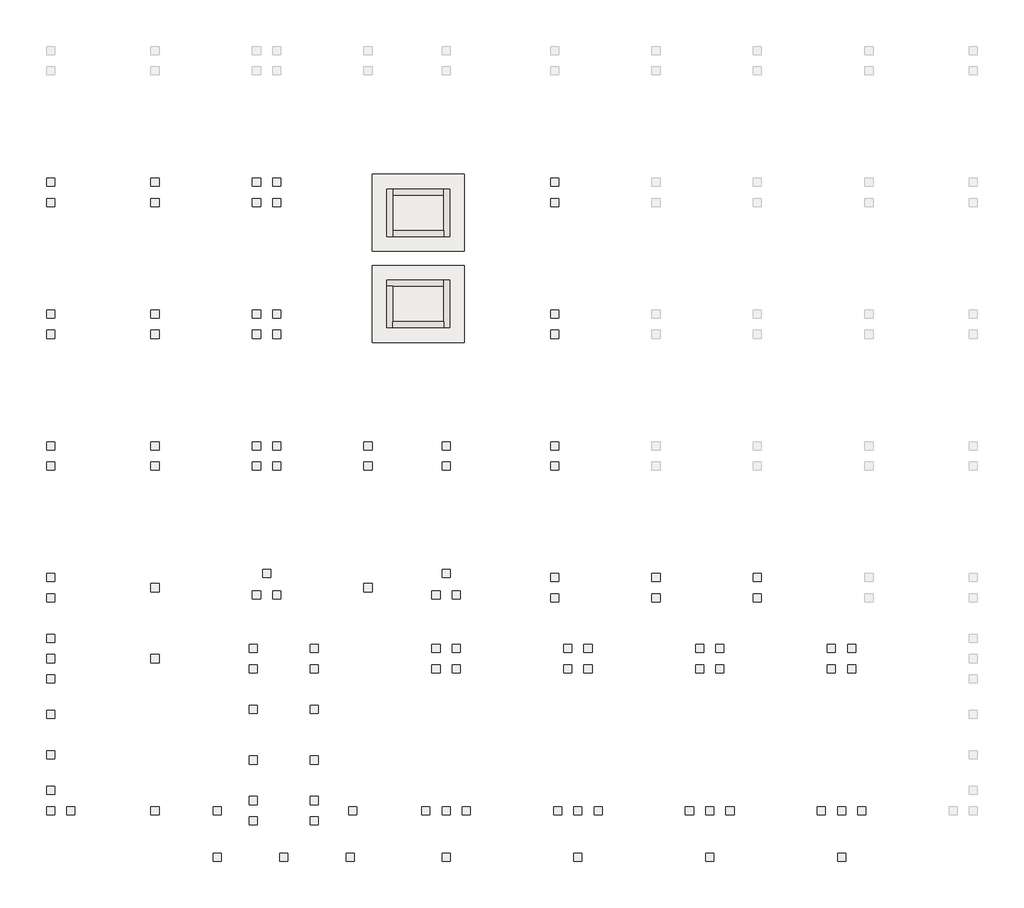
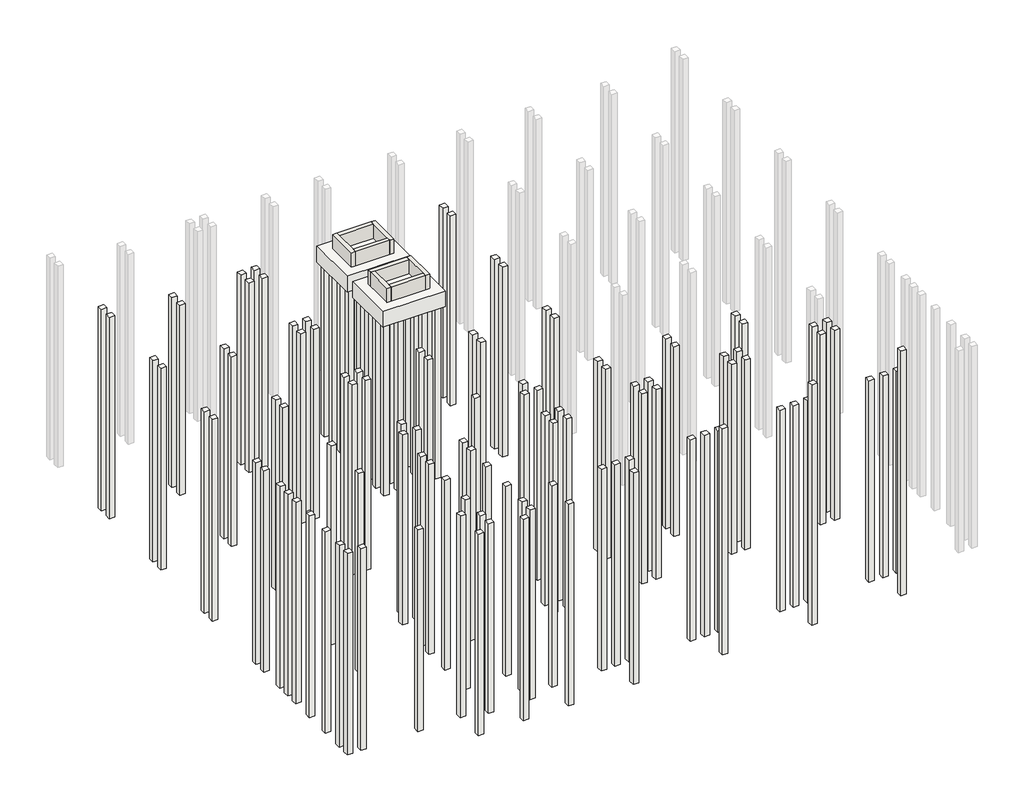
# Not in any storey, part 1 of 2: 143 slabs, 8 walls.
# Revit data of these elements (continued)
# Element 99 (IfcSlab, "NLRS_17_SFO_TLB_funderingspaal geheid beton prefab-AV-MMBPC_gen_rsf : heipaal beton prefab_gen__bxh 400x400") (continued)
#   NLRS_S_draagvermogen_druk = 0.00 kN
#   Angle = 0.00°
#   IsExternal = yes
#   LoadBearing = yes
#   Slanted = 0
#   Phase Created = NLRS_nieuw
#   Materials on its faces: "NLRS_f2_beton prefab_gen_rsf"
# Element 100 (IfcSlab, "NLRS_17_SFO_TLB_funderingspaal geheid beton prefab-AV-MMBPC_gen_rsf : heipaal beton prefab_gen__bxh 400x400")
#   IfcGUID = "3loy75XKz2Rw4dS8JWiaqH"
#   Slanted Angle = 0.00°
#   NLRS_S_draagvermogen_trek = 0.00 kN
#   NLRS_S_draagvermogen_druk = 0.00 kN
#   Angle = 0.00°
#   IsExternal = yes
#   LoadBearing = yes
#   Slanted = 0
#   Phase Created = NLRS_nieuw
#   Materials on its faces: "NLRS_f2_beton prefab_gen_rsf"
# Element 101 (IfcSlab, "NLRS_17_SFO_TLB_funderingspaal geheid beton prefab-AV-MMBPC_gen_rsf : heipaal beton prefab_gen__bxh 400x400")
#   IfcGUID = "3loy75XKz2Rw4dS8JWiaqU"
#   Slanted Angle = 0.00°
#   NLRS_S_draagvermogen_trek = 0.00 kN
#   NLRS_S_draagvermogen_druk = 0.00 kN
#   Angle = 0.00°
#   IsExternal = yes
#   LoadBearing = yes
#   Slanted = 0
#   Phase Created = NLRS_nieuw
#   Materials on its faces: "NLRS_f2_beton prefab_gen_rsf"
# Element 102 (IfcSlab, "NLRS_17_SFO_TLB_funderingspaal geheid beton prefab-AV-MMBPC_gen_rsf : heipaal beton prefab_gen__bxh 400x400")
#   IfcGUID = "3loy75XKz2Rw4dS8JWiaqS"
#   Slanted Angle = 0.00°
#   NLRS_S_draagvermogen_trek = 0.00 kN
#   NLRS_S_draagvermogen_druk = 0.00 kN
#   Angle = 0.00°
#   IsExternal = yes
#   LoadBearing = yes
#   Slanted = 0
#   Phase Created = NLRS_nieuw
#   Materials on its faces: "NLRS_f2_beton prefab_gen_rsf"
# Element 103 (IfcSlab, "NLRS_17_SFO_TLB_funderingspaal geheid beton prefab-AV-MMBPC_gen_rsf : heipaal beton prefab_gen__bxh 400x400")
#   IfcGUID = "3loy75XKz2Rw4dS8JWiaq9"
#   Slanted Angle = 0.00°
#   NLRS_S_draagvermogen_trek = 0.00 kN
#   NLRS_S_draagvermogen_druk = 0.00 kN
#   Angle = 0.00°
#   IsExternal = yes
#   LoadBearing = yes
#   Slanted = 0
#   Phase Created = NLRS_nieuw
#   Materials on its faces: "NLRS_f2_beton prefab_gen_rsf"
# Element 104 (IfcSlab, "NLRS_17_SFO_TLB_funderingspaal geheid beton prefab-AV-MMBPC_gen_rsf : heipaal beton prefab_gen__bxh 400x400")
#   IfcGUID = "3loy75XKz2Rw4dS8JWiaqF"
#   Slanted Angle = 0.00°
#   NLRS_S_draagvermogen_trek = 0.00 kN
#   NLRS_S_draagvermogen_druk = 0.00 kN
#   Angle = 0.00°
#   IsExternal = yes
#   LoadBearing = yes
#   Slanted = 0
#   Phase Created = NLRS_nieuw
#   Materials on its faces: "NLRS_f2_beton prefab_gen_rsf"
# Element 105 (IfcSlab, "NLRS_17_SFO_TLB_funderingspaal geheid beton prefab-AV-MMBPC_gen_rsf : heipaal beton prefab_gen__bxh 400x400")
#   IfcGUID = "3loy75XKz2Rw4dS8JWia7f"
#   Slanted Angle = 0.00°
#   NLRS_S_draagvermogen_trek = 0.00 kN
#   NLRS_S_draagvermogen_druk = 0.00 kN
#   Angle = 0.00°
#   IsExternal = yes
#   LoadBearing = yes
#   Slanted = 0
#   Phase Created = NLRS_nieuw
#   Materials on its faces: "NLRS_f2_beton prefab_gen_rsf"
# Element 106 (IfcSlab, "NLRS_17_SFO_TLB_funderingspaal geheid beton prefab-AV-MMBPC_gen_rsf : heipaal beton prefab_gen__bxh 400x400")
#   IfcGUID = "3loy75XKz2Rw4dS8JWia6M"
#   Slanted Angle = 0.00°
#   NLRS_S_draagvermogen_trek = 0.00 kN
#   NLRS_S_draagvermogen_druk = 0.00 kN
#   Angle = 0.00°
#   IsExternal = yes
#   LoadBearing = yes
#   Slanted = 0
#   Phase Created = NLRS_nieuw
#   Materials on its faces: "NLRS_f2_beton prefab_gen_rsf"
# Element 107 (IfcSlab, "NLRS_17_SFO_TLB_funderingspaal geheid beton prefab-AV-MMBPC_gen_rsf : heipaal beton prefab_gen__bxh 400x400")
#   IfcGUID = "3loy75XKz2Rw4dS8JWiaPz"
#   Slanted Angle = 0.00°
#   NLRS_S_draagvermogen_trek = 0.00 kN
#   NLRS_S_draagvermogen_druk = 0.00 kN
#   Angle = 0.00°
#   IsExternal = yes
#   LoadBearing = yes
#   Slanted = 0
#   Phase Created = NLRS_nieuw
#   Materials on its faces: "NLRS_f2_beton prefab_gen_rsf"
# Element 108 (IfcSlab, "NLRS_17_SFO_TLB_funderingspaal geheid beton prefab-AV-MMBPC_gen_rsf : heipaal beton prefab_gen__bxh 400x400")
#   IfcGUID = "3yoae3mAzBRekDMiYpsxUC"
#   Slanted Angle = 0.00°
#   NLRS_S_draagvermogen_trek = 0.00 kN
#   NLRS_S_draagvermogen_druk = 0.00 kN
#   Angle = 0.00°
#   IsExternal = yes
#   LoadBearing = yes
#   Slanted = 0
#   Phase Created = NLRS_nieuw
#   Materials on its faces: "NLRS_f2_beton prefab_gen_rsf"
# Element 109 (IfcSlab, "NLRS_17_SFO_TLB_funderingspaal geheid beton prefab-AV-MMBPC_gen_rsf : heipaal beton prefab_gen__bxh 400x400")
#   IfcGUID = "3yoae3mAzBRekDMiYpsxUN"
#   Slanted Angle = 0.00°
#   NLRS_S_draagvermogen_trek = 0.00 kN
#   NLRS_S_draagvermogen_druk = 0.00 kN
#   Angle = 0.00°
#   IsExternal = yes
#   LoadBearing = yes
#   Slanted = 0
#   Phase Created = NLRS_nieuw
#   Materials on its faces: "NLRS_f2_beton prefab_gen_rsf"
# Element 110 (IfcSlab, "NLRS_17_SFO_TLB_funderingspaal geheid beton prefab-AV-MMBPC_gen_rsf : heipaal beton prefab_gen__bxh 400x400")
#   IfcGUID = "3yoae3mAzBRekDMiYpsxUU"
#   Slanted Angle = 0.00°
#   NLRS_S_draagvermogen_trek = 0.00 kN
#   NLRS_S_draagvermogen_druk = 0.00 kN
#   Angle = 0.00°
#   IsExternal = yes
#   LoadBearing = yes
#   Slanted = 0
#   Phase Created = NLRS_nieuw
#   Materials on its faces: "NLRS_f2_beton prefab_gen_rsf"
# Element 111 (IfcSlab, "NLRS_17_SFO_TLB_funderingspaal geheid beton prefab-AV-MMBPC_gen_rsf : heipaal beton prefab_gen__bxh 400x400")
#   IfcGUID = "3yoae3mAzBRekDMiYpsxVf"
#   Slanted Angle = 0.00°
#   NLRS_S_draagvermogen_trek = 0.00 kN
#   NLRS_S_draagvermogen_druk = 0.00 kN
#   Angle = 0.00°
#   IsExternal = yes
#   LoadBearing = yes
#   Slanted = 0
#   Phase Created = NLRS_nieuw
#   Materials on its faces: "NLRS_f2_beton prefab_gen_rsf"
# Element 112 (IfcSlab, "NLRS_17_SFO_TLB_funderingspaal geheid beton prefab-AV-MMBPC_gen_rsf : heipaal beton prefab_gen__bxh 400x400")
#   IfcGUID = "22y6L5gAz9AR8RjJaZzOrs"
#   Slanted Angle = 0.00°
#   NLRS_S_draagvermogen_trek = 0.00 kN
#   NLRS_S_draagvermogen_druk = 0.00 kN
#   Angle = 0.00°
#   IsExternal = yes
#   LoadBearing = yes
#   Slanted = 0
#   Phase Created = NLRS_nieuw
#   Materials on its faces: "NLRS_f2_beton prefab_gen_rsf"
# Element 113 (IfcSlab, "NLRS_17_SFO_TLB_funderingspaal geheid beton prefab-AV-MMBPC_gen_rsf : heipaal beton prefab_gen__bxh 400x400")
#   IfcGUID = "22y6L5gAz9AR8RjJaZzOqH"
#   Slanted Angle = 0.00°
#   NLRS_S_draagvermogen_trek = 0.00 kN
#   NLRS_S_draagvermogen_druk = 0.00 kN
#   Angle = 0.00°
#   IsExternal = yes
#   LoadBearing = yes
#   Slanted = 0
#   Phase Created = NLRS_nieuw
#   Materials on its faces: "NLRS_f2_beton prefab_gen_rsf"
# Element 114 (IfcSlab, "NLRS_17_SFO_TLB_funderingspaal geheid beton prefab-AV-MMBPC_gen_rsf : heipaal beton prefab_gen__bxh 400x400")
#   IfcGUID = "22y6L5gAz9AR8RjJaZzOo$"
#   Slanted Angle = 0.00°
#   NLRS_S_draagvermogen_trek = 0.00 kN
#   NLRS_S_draagvermogen_druk = 0.00 kN
#   Angle = 0.00°
#   IsExternal = yes
#   LoadBearing = yes
#   Slanted = 0
#   Phase Created = NLRS_nieuw
#   Materials on its faces: "NLRS_f2_beton prefab_gen_rsf"
# Element 115 (IfcSlab, "NLRS_17_SFO_TLB_funderingspaal geheid beton prefab-AV-MMBPC_gen_rsf : heipaal beton prefab_gen__bxh 400x400")
#   IfcGUID = "22y6L5gAz9AR8RjJaZzOn6"
#   Slanted Angle = 0.00°
#   NLRS_S_draagvermogen_trek = 0.00 kN
#   NLRS_S_draagvermogen_druk = 0.00 kN
#   Angle = 0.00°
#   IsExternal = yes
#   LoadBearing = yes
#   Slanted = 0
#   Phase Created = NLRS_nieuw
#   Materials on its faces: "NLRS_f2_beton prefab_gen_rsf"
# Element 116 (IfcSlab, "NLRS_17_SFO_TLB_funderingspaal geheid beton prefab-AV-MMBPC_gen_rsf : heipaal beton prefab_gen__bxh 400x400")
#   IfcGUID = "22y6L5gAz9AR8RjJaZzOmJ"
#   Slanted Angle = 0.00°
#   NLRS_S_draagvermogen_trek = 0.00 kN
#   NLRS_S_draagvermogen_druk = 0.00 kN
#   Angle = 0.00°
#   IsExternal = yes
#   LoadBearing = yes
#   Slanted = 0
#   Phase Created = NLRS_nieuw
#   Materials on its faces: "NLRS_f2_beton prefab_gen_rsf"
# Element 117 (IfcSlab, "NLRS_17_SFO_TLB_funderingspaal geheid beton prefab-AV-MMBPC_gen_rsf : heipaal beton prefab_gen__bxh 400x400")
#   IfcGUID = "22y6L5gAz9AR8RjJaZzOmD"
#   Slanted Angle = 0.00°
#   NLRS_S_draagvermogen_trek = 0.00 kN
#   NLRS_S_draagvermogen_druk = 0.00 kN
#   Angle = 0.00°
#   IsExternal = yes
#   LoadBearing = yes
#   Slanted = 0
#   Phase Created = NLRS_nieuw
#   Materials on its faces: "NLRS_f2_beton prefab_gen_rsf"
# Element 118 (IfcSlab, "NLRS_17_SFO_TLB_funderingspaal geheid beton prefab-AV-MMBPC_gen_rsf : heipaal beton prefab_gen__bxh 400x400")
#   IfcGUID = "22y6L5gAz9AR8RjJaZzOmk"
#   Slanted Angle = 0.00°
#   NLRS_S_draagvermogen_trek = 0.00 kN
#   NLRS_S_draagvermogen_druk = 0.00 kN
#   Angle = 0.00°
#   IsExternal = yes
#   LoadBearing = yes
#   Slanted = 0
#   Phase Created = NLRS_nieuw
#   Materials on its faces: "NLRS_f2_beton prefab_gen_rsf"
# Element 119 (IfcSlab, "NLRS_17_SFO_TLB_funderingspaal geheid beton prefab-AV-MMBPC_gen_rsf : heipaal beton prefab_gen__bxh 400x400")
#   IfcGUID = "22y6L5gAz9AR8RjJaZzOme"
#   Slanted Angle = 0.00°
#   NLRS_S_draagvermogen_trek = 0.00 kN
#   NLRS_S_draagvermogen_druk = 0.00 kN
#   Angle = 0.00°
#   IsExternal = yes
#   LoadBearing = yes
#   Slanted = 0
#   Phase Created = NLRS_nieuw
#   Materials on its faces: "NLRS_f2_beton prefab_gen_rsf"
# Element 120 (IfcSlab, "NLRS_17_SFO_TLB_funderingspaal geheid beton prefab-AV-MMBPC_gen_rsf : heipaal beton prefab_gen__bxh 400x400")
#   IfcGUID = "22y6L5gAz9AR8RjJaZzO$2"
#   Slanted Angle = 0.00°
#   NLRS_S_draagvermogen_trek = 0.00 kN
#   NLRS_S_draagvermogen_druk = 0.00 kN
#   Angle = 0.00°
#   IsExternal = yes
#   LoadBearing = yes
#   Slanted = 0
#   Phase Created = NLRS_nieuw
#   Materials on its faces: "NLRS_f2_beton prefab_gen_rsf"
# Element 121 (IfcSlab, "NLRS_17_SFO_TLB_funderingspaal geheid beton prefab-AV-MMBPC_gen_rsf : heipaal beton prefab_gen__bxh 400x400")
#   IfcGUID = "22y6L5gAz9AR8RjJaZzO$y"
#   Slanted Angle = 0.00°
#   NLRS_S_draagvermogen_trek = 0.00 kN
#   NLRS_S_draagvermogen_druk = 0.00 kN
#   Angle = 0.00°
#   IsExternal = yes
#   LoadBearing = yes
#   Slanted = 0
#   Phase Created = NLRS_nieuw
#   Materials on its faces: "NLRS_f2_beton prefab_gen_rsf"
# Element 122 (IfcSlab, "NLRS_17_SFO_TLB_funderingspaal geheid beton prefab-AV-MMBPC_gen_rsf : heipaal beton prefab_gen__bxh 400x400")
#   IfcGUID = "22y6L5gAz9AR8RjJaZzO$_"
#   Slanted Angle = 0.00°
#   NLRS_S_draagvermogen_trek = 0.00 kN
#   NLRS_S_draagvermogen_druk = 0.00 kN
#   Angle = 0.00°
#   IsExternal = yes
#   LoadBearing = yes
#   Slanted = 0
#   Phase Created = NLRS_nieuw
#   Materials on its faces: "NLRS_f2_beton prefab_gen_rsf"
# Element 123 (IfcSlab, "NLRS_17_SFO_TLB_funderingspaal geheid beton prefab-AV-MMBPC_gen_rsf : heipaal beton prefab_gen__bxh 400x400")
#   IfcGUID = "22y6L5gAz9AR8RjJaZzO$u"
#   Slanted Angle = 0.00°
#   NLRS_S_draagvermogen_trek = 0.00 kN
#   NLRS_S_draagvermogen_druk = 0.00 kN
#   Angle = 0.00°
#   IsExternal = yes
#   LoadBearing = yes
#   Slanted = 0
#   Phase Created = NLRS_nieuw
#   Materials on its faces: "NLRS_f2_beton prefab_gen_rsf"
# Element 124 (IfcSlab, "NLRS_17_SFO_TLB_funderingspaal geheid beton prefab-AV-MMBPC_gen_rsf : heipaal beton prefab_gen__bxh 400x400")
#   IfcGUID = "22y6L5gAz9AR8RjJaZzO$w"
#   Slanted Angle = 0.00°
#   NLRS_S_draagvermogen_trek = 0.00 kN
#   NLRS_S_draagvermogen_druk = 0.00 kN
#   Angle = 0.00°
#   IsExternal = yes
#   LoadBearing = yes
#   Slanted = 0
#   Phase Created = NLRS_nieuw
#   Materials on its faces: "NLRS_f2_beton prefab_gen_rsf"
# Element 125 (IfcSlab, "NLRS_17_SFO_TLB_funderingspaal geheid beton prefab-AV-MMBPC_gen_rsf : heipaal beton prefab_gen__bxh 400x400")
#   IfcGUID = "22y6L5gAz9AR8RjJaZzO$q"
#   Slanted Angle = 0.00°
#   NLRS_S_draagvermogen_trek = 0.00 kN
#   NLRS_S_draagvermogen_druk = 0.00 kN
#   Angle = 0.00°
#   IsExternal = yes
#   LoadBearing = yes
#   Slanted = 0
#   Phase Created = NLRS_nieuw
#   Materials on its faces: "NLRS_f2_beton prefab_gen_rsf"
# Element 126 (IfcSlab, "NLRS_17_SFO_TLB_funderingspaal geheid beton prefab-AV-MMBPC_gen_rsf : heipaal beton prefab_gen__bxh 400x400")
#   IfcGUID = "22y6L5gAz9AR8RjJaZzO$s"
#   Slanted Angle = 0.00°
#   NLRS_S_draagvermogen_trek = 0.00 kN
#   NLRS_S_draagvermogen_druk = 0.00 kN
#   Angle = 0.00°
#   IsExternal = yes
#   LoadBearing = yes
#   Slanted = 0
#   Phase Created = NLRS_nieuw
#   Materials on its faces: "NLRS_f2_beton prefab_gen_rsf"
# Element 127 (IfcSlab, "NLRS_17_SFO_TLB_funderingspaal geheid beton prefab-AV-MMBPC_gen_rsf : heipaal beton prefab_gen__bxh 400x400")
#   IfcGUID = "22y6L5gAz9AR8RjJaZzO$m"
#   Slanted Angle = 0.00°
#   NLRS_S_draagvermogen_trek = 0.00 kN
#   NLRS_S_draagvermogen_druk = 0.00 kN
#   Angle = 0.00°
#   IsExternal = yes
#   LoadBearing = yes
#   Slanted = 0
#   Phase Created = NLRS_nieuw
#   Materials on its faces: "NLRS_f2_beton prefab_gen_rsf"
# Element 128 (IfcSlab, "NLRS_17_SFO_TLB_funderingspaal geheid beton prefab-AV-MMBPC_gen_rsf : heipaal beton prefab_gen__bxh 400x400")
#   IfcGUID = "22y6L5gAz9AR8RjJaZzOuC"
#   Slanted Angle = 0.00°
#   NLRS_S_draagvermogen_trek = 0.00 kN
#   NLRS_S_draagvermogen_druk = 0.00 kN
#   Angle = 0.00°
#   IsExternal = yes
#   LoadBearing = yes
#   Slanted = 0
#   Phase Created = NLRS_nieuw
#   Materials on its faces: "NLRS_f2_beton prefab_gen_rsf"
# Element 129 (IfcSlab, "NLRS_17_SFO_TLB_funderingspaal geheid beton prefab-AV-MMBPC_gen_rsf : heipaal beton prefab_gen__bxh 400x400")
#   IfcGUID = "22y6L5gAz9AR8RjJaZzOuE"
#   Slanted Angle = 0.00°
#   NLRS_S_draagvermogen_trek = 0.00 kN
#   NLRS_S_draagvermogen_druk = 0.00 kN
#   Angle = 0.00°
#   IsExternal = yes
#   LoadBearing = yes
#   Slanted = 0
#   Phase Created = NLRS_nieuw
#   Materials on its faces: "NLRS_f2_beton prefab_gen_rsf"
# Element 130 (IfcSlab, "NLRS_17_SFO_TLB_funderingspaal geheid beton prefab-AV-MMBPC_gen_rsf : heipaal beton prefab_gen__bxh 400x400")
#   IfcGUID = "22y6L5gAz9AR8RjJaZzOu8"
#   Slanted Angle = 0.00°
#   NLRS_S_draagvermogen_trek = 0.00 kN
#   NLRS_S_draagvermogen_druk = 0.00 kN
#   Angle = 0.00°
#   IsExternal = yes
#   LoadBearing = yes
#   Slanted = 0
#   Phase Created = NLRS_nieuw
#   Materials on its faces: "NLRS_f2_beton prefab_gen_rsf"
# Element 131 (IfcSlab, "NLRS_17_SFO_TLB_funderingspaal geheid beton prefab-AV-MMBPC_gen_rsf : heipaal beton prefab_gen__bxh 400x400")
#   IfcGUID = "22y6L5gAz9AR8RjJaZzOuA"
#   Slanted Angle = 0.00°
#   NLRS_S_draagvermogen_trek = 0.00 kN
#   NLRS_S_draagvermogen_druk = 0.00 kN
#   Angle = 0.00°
#   IsExternal = yes
#   LoadBearing = yes
#   Slanted = 0
#   Phase Created = NLRS_nieuw
#   Materials on its faces: "NLRS_f2_beton prefab_gen_rsf"
# Element 132 (IfcSlab, "NLRS_17_SFO_TLB_funderingspaal geheid beton prefab-AV-MMBPC_gen_rsf : heipaal beton prefab_gen__bxh 400x400")
#   IfcGUID = "22y6L5gAz9AR8RjJaZzOu4"
#   Slanted Angle = 0.00°
#   NLRS_S_draagvermogen_trek = 0.00 kN
#   NLRS_S_draagvermogen_druk = 0.00 kN
#   Angle = 0.00°
#   IsExternal = yes
#   LoadBearing = yes
#   Slanted = 0
#   Phase Created = NLRS_nieuw
#   Materials on its faces: "NLRS_f2_beton prefab_gen_rsf"
# Element 133 (IfcSlab, "NLRS_17_SFO_TLB_funderingspaal geheid beton prefab-AV-MMBPC_gen_rsf : heipaal beton prefab_gen__bxh 400x400")
#   IfcGUID = "22y6L5gAz9AR8RjJaZzOu6"
#   Slanted Angle = 0.00°
#   NLRS_S_draagvermogen_trek = 0.00 kN
#   NLRS_S_draagvermogen_druk = 0.00 kN
#   Angle = 0.00°
#   IsExternal = yes
#   LoadBearing = yes
#   Slanted = 0
#   Phase Created = NLRS_nieuw
#   Materials on its faces: "NLRS_f2_beton prefab_gen_rsf"
# Element 134 (IfcSlab, "NLRS_17_SFO_TLB_funderingspaal geheid beton prefab-AV-MMBPC_gen_rsf : heipaal beton prefab_gen__bxh 400x400")
#   IfcGUID = "22y6L5gAz9AR8RjJaZzOu0"
#   Slanted Angle = 0.00°
#   NLRS_S_draagvermogen_trek = 0.00 kN
#   NLRS_S_draagvermogen_druk = 0.00 kN
#   Angle = 0.00°
#   IsExternal = yes
#   LoadBearing = yes
#   Slanted = 0
#   Phase Created = NLRS_nieuw
#   Materials on its faces: "NLRS_f2_beton prefab_gen_rsf"
# Element 135 (IfcSlab, "NLRS_17_SFO_TLB_funderingspaal geheid beton prefab-AV-MMBPC_gen_rsf : heipaal beton prefab_gen__bxh 400x400")
#   IfcGUID = "22y6L5gAz9AR8RjJaZzOu2"
#   Slanted Angle = 0.00°
#   NLRS_S_draagvermogen_trek = 0.00 kN
#   NLRS_S_draagvermogen_druk = 0.00 kN
#   Angle = 0.00°
#   IsExternal = yes
#   LoadBearing = yes
#   Slanted = 0
#   Phase Created = NLRS_nieuw
#   Materials on its faces: "NLRS_f2_beton prefab_gen_rsf"
# Element 136 (IfcSlab, "NLRS_17_SFO_TLB_funderingspaal geheid beton prefab-AV-MMBPC_gen_rsf : heipaal beton prefab_gen__bxh 400x400")
#   IfcGUID = "22y6L5gAz9AR8RjJaZzOuy"
#   Slanted Angle = 0.00°
#   NLRS_S_draagvermogen_trek = 0.00 kN
#   NLRS_S_draagvermogen_druk = 0.00 kN
#   Angle = 0.00°
#   IsExternal = yes
#   LoadBearing = yes
#   Slanted = 0
#   Phase Created = NLRS_nieuw
#   Materials on its faces: "NLRS_f2_beton prefab_gen_rsf"
# Element 137 (IfcSlab, "NLRS_17_SFO_TLB_funderingspaal geheid beton prefab-AV-MMBPC_gen_rsf : heipaal beton prefab_gen__bxh 400x400")
#   IfcGUID = "22y6L5gAz9AR8RjJaZzOu_"
#   Slanted Angle = 0.00°
#   NLRS_S_draagvermogen_trek = 0.00 kN
#   NLRS_S_draagvermogen_druk = 0.00 kN
#   Angle = 0.00°
#   IsExternal = yes
#   LoadBearing = yes
#   Slanted = 0
#   Phase Created = NLRS_nieuw
#   Materials on its faces: "NLRS_f2_beton prefab_gen_rsf"
# Element 138 (IfcSlab, "NLRS_17_SFO_TLB_funderingspaal geheid beton prefab-AV-MMBPC_gen_rsf : heipaal beton prefab_gen__bxh 400x400")
#   IfcGUID = "22y6L5gAz9AR8RjJaZzOuu"
#   Slanted Angle = 0.00°
#   NLRS_S_draagvermogen_trek = 0.00 kN
#   NLRS_S_draagvermogen_druk = 0.00 kN
#   Angle = 0.00°
#   IsExternal = yes
#   LoadBearing = yes
#   Slanted = 0
#   Phase Created = NLRS_nieuw
#   Materials on its faces: "NLRS_f2_beton prefab_gen_rsf"
# Element 139 (IfcSlab, "NLRS_17_SFO_TLB_funderingspaal geheid beton prefab-AV-MMBPC_gen_rsf : heipaal beton prefab_gen__bxh 400x400")
#   IfcGUID = "22y6L5gAz9AR8RjJaZzOuw"
#   Slanted Angle = 0.00°
#   NLRS_S_draagvermogen_trek = 0.00 kN
#   NLRS_S_draagvermogen_druk = 0.00 kN
#   Angle = 0.00°
#   IsExternal = yes
#   LoadBearing = yes
#   Slanted = 0
#   Phase Created = NLRS_nieuw
#   Materials on its faces: "NLRS_f2_beton prefab_gen_rsf"
# Element 140 (IfcSlab, "NLRS_17_SFO_TLB_funderingspaal geheid beton prefab-AV-MMBPC_gen_rsf : heipaal beton prefab_gen__bxh 400x400")
#   IfcGUID = "22y6L5gAz9AR8RjJaZzOuq"
#   Slanted Angle = 0.00°
#   NLRS_S_draagvermogen_trek = 0.00 kN
#   NLRS_S_draagvermogen_druk = 0.00 kN
#   Angle = 0.00°
#   IsExternal = yes
#   LoadBearing = yes
#   Slanted = 0
#   Phase Created = NLRS_nieuw
#   Materials on its faces: "NLRS_f2_beton prefab_gen_rsf"
# Element 141 (IfcSlab, "NLRS_17_SFO_TLB_funderingspaal geheid beton prefab-AV-MMBPC_gen_rsf : heipaal beton prefab_gen__bxh 400x400")
#   IfcGUID = "22y6L5gAz9AR8RjJaZzOus"
#   Slanted Angle = 0.00°
#   NLRS_S_draagvermogen_trek = 0.00 kN
#   NLRS_S_draagvermogen_druk = 0.00 kN
#   Angle = 0.00°
#   IsExternal = yes
#   LoadBearing = yes
#   Slanted = 0
#   Phase Created = NLRS_nieuw
#   Materials on its faces: "NLRS_f2_beton prefab_gen_rsf"
# Element 142 (IfcSlab, "NLRS_17_SFO_TLB_funderingspaal geheid beton prefab-AV-MMBPC_gen_rsf : heipaal beton prefab_gen__bxh 400x400")
#   IfcGUID = "22y6L5gAz9AR8RjJaZzOum"
#   Slanted Angle = 0.00°
#   NLRS_S_draagvermogen_trek = 0.00 kN
#   NLRS_S_draagvermogen_druk = 0.00 kN
#   Angle = 0.00°
#   IsExternal = yes
#   LoadBearing = yes
#   Slanted = 0
#   Phase Created = NLRS_nieuw
#   Materials on its faces: "NLRS_f2_beton prefab_gen_rsf"
# Element 143 (IfcSlab, "NLRS_17_SFO_TLB_funderingspaal geheid beton prefab-AV-MMBPC_gen_rsf : heipaal beton prefab_gen__bxh 400x400")
#   IfcGUID = "22y6L5gAz9AR8RjJaZzOuo"
#   Slanted Angle = 0.00°
#   NLRS_S_draagvermogen_trek = 0.00 kN
#   NLRS_S_draagvermogen_druk = 0.00 kN
#   Angle = 0.00°
#   IsExternal = yes
#   LoadBearing = yes
#   Slanted = 0
#   Phase Created = NLRS_nieuw
#   Materials on its faces: "NLRS_f2_beton prefab_gen_rsf"
# Element 144 (IfcWall, "NLRS_16_WA_beton ihw 300_gen_rsf")
#   IfcGUID = "22y6L5gAz9AR8RjJaZzOY4"
#   Comments = ""
#   Top Offset = 0 mm
#   Base Offset = 0 mm
#   wall height = 1100 mm
#   IsExternal = yes
#   LoadBearing = yes
#   Phase Created = NLRS_nieuw
#   Base Constraint = -02_bk ruwe vloer liftput
#   Top Constraint = -01_ok ruwe vloer
#   Materials on its faces: "NLRS_f2_beton ihwg_gen_rsf"
# Element 145 (IfcWall, "NLRS_16_WA_beton ihw 300_gen_rsf")
#   IfcGUID = "22y6L5gAz9AR8RjJaZzOY6"
#   Comments = ""
#   Top Offset = 0 mm
#   Base Offset = 0 mm
#   wall height = 1100 mm
#   IsExternal = yes
#   LoadBearing = yes
#   Phase Created = NLRS_nieuw
#   Base Constraint = -02_bk ruwe vloer liftput
#   Top Constraint = -01_ok ruwe vloer
#   Materials on its faces: "NLRS_f2_beton ihwg_gen_rsf"
# Element 146 (IfcWall, "NLRS_16_WA_beton ihw 300_gen_rsf")
#   IfcGUID = "22y6L5gAz9AR8RjJaZzOY0"
#   Comments = ""
#   Top Offset = 0 mm
#   Base Offset = 0 mm
#   wall height = 1100 mm
#   IsExternal = yes
#   LoadBearing = yes
#   Phase Created = NLRS_nieuw
#   Base Constraint = -02_bk ruwe vloer liftput
#   Top Constraint = -01_ok ruwe vloer
#   Materials on its faces: "NLRS_f2_beton ihwg_gen_rsf"
# Element 147 (IfcWall, "NLRS_16_WA_beton ihw 300_gen_rsf")
#   IfcGUID = "22y6L5gAz9AR8RjJaZzOY2"
#   Comments = ""
#   Top Offset = 0 mm
#   Base Offset = 0 mm
#   wall height = 1100 mm
#   IsExternal = yes
#   LoadBearing = yes
#   Phase Created = NLRS_nieuw
#   Base Constraint = -02_bk ruwe vloer liftput
#   Top Constraint = -01_ok ruwe vloer
#   Materials on its faces: "NLRS_f2_beton ihwg_gen_rsf"
# Element 148 (IfcWall, "NLRS_16_WA_beton ihw 300_gen_rsf")
#   IfcGUID = "22y6L5gAz9AR8RjJaZzOYy"
#   Comments = ""
#   Top Offset = 0 mm
#   Base Offset = 0 mm
#   wall height = 1100 mm
#   IsExternal = yes
#   LoadBearing = yes
#   Phase Created = NLRS_nieuw
#   Base Constraint = -02_bk ruwe vloer liftput
#   Top Constraint = -01_ok ruwe vloer
#   Materials on its faces: "NLRS_f2_beton ihwg_gen_rsf"
# Element 149 (IfcWall, "NLRS_16_WA_beton ihw 300_gen_rsf")
#   IfcGUID = "22y6L5gAz9AR8RjJaZzOY_"
#   Comments = ""
#   Top Offset = 0 mm
#   Base Offset = 0 mm
#   wall height = 1100 mm
#   IsExternal = yes
#   LoadBearing = yes
#   Phase Created = NLRS_nieuw
#   Base Constraint = -02_bk ruwe vloer liftput
#   Top Constraint = -01_ok ruwe vloer
#   Materials on its faces: "NLRS_f2_beton ihwg_gen_rsf"
# Element 150 (IfcWall, "NLRS_16_WA_beton ihw 300_gen_rsf")
#   IfcGUID = "22y6L5gAz9AR8RjJaZzOYu"
#   Comments = ""
#   Top Offset = 0 mm
#   Base Offset = 0 mm
#   wall height = 1100 mm
#   IsExternal = yes
#   LoadBearing = yes
#   Phase Created = NLRS_nieuw
#   Base Constraint = -02_bk ruwe vloer liftput
#   Top Constraint = -01_ok ruwe vloer
#   Materials on its faces: "NLRS_f2_beton ihwg_gen_rsf"
# Element 151 (IfcWall, "NLRS_16_WA_beton ihw 300_gen_rsf")
#   IfcGUID = "22y6L5gAz9AR8RjJaZzOYw"
#   Comments = ""
#   Top Offset = 0 mm
#   Base Offset = 0 mm
#   wall height = 1100 mm
#   IsExternal = yes
#   LoadBearing = yes
#   Phase Created = NLRS_nieuw
#   Base Constraint = -02_bk ruwe vloer liftput
#   Top Constraint = -01_ok ruwe vloer
#   Materials on its faces: "NLRS_f2_beton ihwg_gen_rsf"
# Materials
#   "NLRS_f2_beton ihwg_gen_rsf": class "F - Niet gebakken kunststeen", colour RGB 129 133 118, transparency 0, Keynote = "f2", Manufacturer = "Revit Standards Foundation", URL = "www.revitstandards.org", Description = "beton ihwg", Cost = 0
#   "NLRS_f2_beton prefab_gen_rsf": class "F - Niet gebakken kunststeen", colour RGB 129 133 118, transparency 0, Keynote = "f2", Manufacturer = "Revit Standards Foundation", URL = "www.revitstandards.org", Description = "beton prefab", Cost = 0
